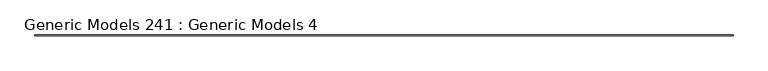
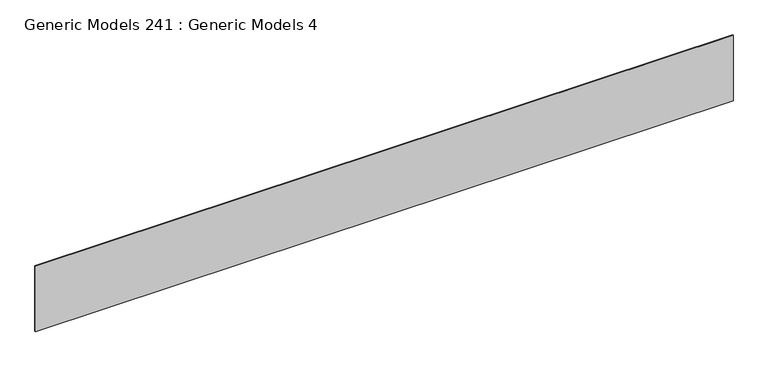
"""IFC4 building model written with IfcOpenShell, lengths in millimetres: proxy geometry, Generic Models 241 : Generic Models 4."""

from ifc_helpers import new_model, si_unit, frame, origin, place, context, project, spatial, polyline, outline, extrude, source, transform, mapped, element, save


def generic_models_241_generic_models_4_ea583cd8(model_context):
    return source(origin(), model_context, "Body", "SweptSolid", [
        extrude(outline(polyline([(-2152.1733045, -29089.2060818), (-2152.1733045, -29108.2560818), (-20795.7733045, -29108.2560818), (-20795.7733045, -29089.2060818), (-2152.1733045, -29089.2060818)])), frame((0.0, 0.0, 126163.227214), z_axis=(0.0, 0.0, 1.0), x_axis=(1.0, 0.0, 0.0)), (0.0, 0.0, 1.0), 1847.85),
    ])


if __name__ == "__main__":
    model = new_model("IFC4")
    model_context = context("Model", 3, world=origin())
    ifc_project = project(units=[si_unit("LENGTHUNIT", "METRE", prefix="MILLI")], contexts=[model_context])
    site = spatial("IfcSite", under=ifc_project)
    building = spatial("IfcBuilding", under=site)
    placement = place(None, origin())
    generic_models_241_generic_models_4_shape = generic_models_241_generic_models_4_ea583cd8(model_context)
    element("IfcBuildingElementProxy", 1, Name="Generic Models 241 : Generic Models 4", ObjectType="Generic Models 241 : Generic Models 4", at=placement, inside=building, context=model_context, shape_type="MappedRepresentation", body=[
        mapped(generic_models_241_generic_models_4_shape, transform((0.0, 0.0, 0.0), x_axis=(1.0, 0.0, 0.0), y_axis=(0.0, 1.0, 0.0), z_axis=(0.0, 0.0, 1.0))),
    ])
    save(model, "model.ifc")

# Revit data of these elements
# Element 1 (IfcBuildingElementProxy, "Generic Models 241 : Generic Models 4")
#   Materials on its faces: "_CDX PLYWOOD - SEE STRUCT DWGs"
# Materials
#   "_CDX PLYWOOD - SEE STRUCT DWGs": class "Generic", colour RGB 98 75 74, transparency 0, Cost = 0
